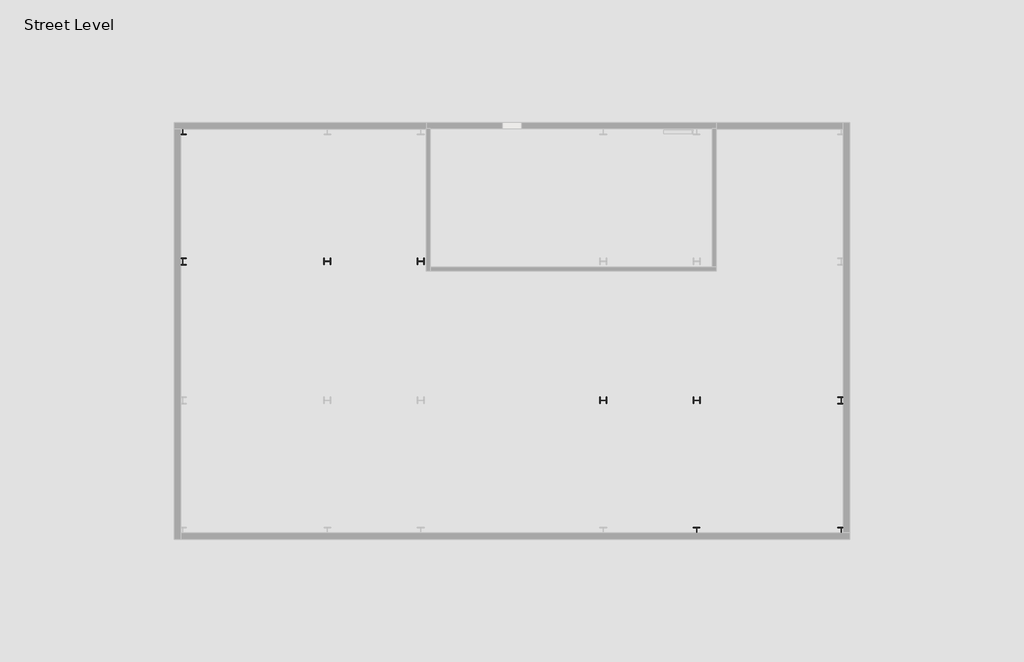
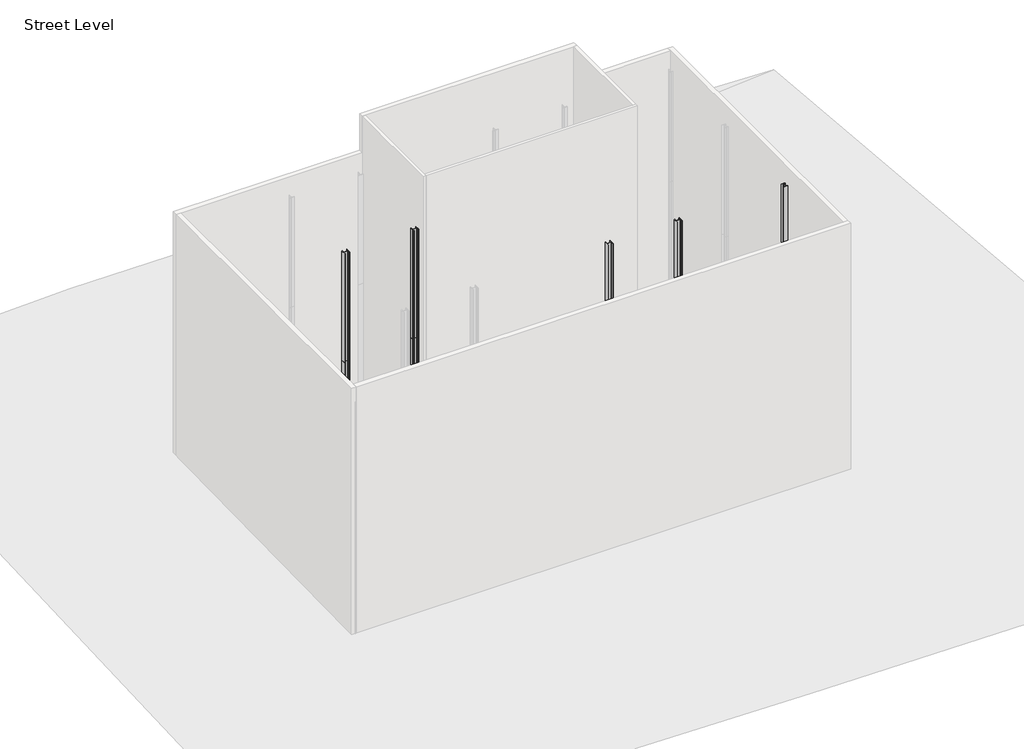
# One storey, part 2 of 3: 9 columns.
"""IFC4 building model written with IfcOpenShell, lengths in millimetres."""

from ifc_helpers import new_model, si_unit, point, frame, frame_2d, origin, place, context, project, spatial, polyline, circle_curve, trimmed, segment, composite_curve, outline, extrude, element, save

model = new_model("IFC4")

# Units and contexts
model_context = context("Model", 3, world=origin())
ifc_project = project(units=[si_unit("LENGTHUNIT", "METRE", prefix="MILLI")], contexts=[model_context])

# Site, building, storey
site = spatial("IfcSite", under=ifc_project)
building = spatial("IfcBuilding", under=site)
storey = spatial("IfcBuildingStorey", under=building, Name="Street Level", Elevation=-914.4)

# Columns
placement = place(None, origin())
element("IfcColumn", 1, ObjectType="W-Wide Flange-Column : W12X87", at=placement, inside=storey, context=model_context, shape_type="SweptSolid", body=[
    extrude(outline(composite_curve([segment(polyline([(3260.1377268, -3562.1684696), (3239.5637268, -3562.1684696), (3239.5637268, -3437.3274696)]), True, "CONTINUOUS"), segment(trimmed(circle_curve(frame_2d((3217.2752268, -3437.3274696)), 22.2885), [point((3239.5637268, -3437.3274696))], [point((3217.2752268, -3415.0389696))], True, "CARTESIAN"), True, "CONTINUOUS"), segment(polyline([(3217.2752268, -3415.0389696), (2985.5002268, -3415.0389696)]), True, "CONTINUOUS"), segment(trimmed(circle_curve(frame_2d((2985.5002268, -3437.3274696)), 22.2885), [point((2985.5002268, -3415.0389696))], [point((2963.2117268, -3437.3274696))], True, "CARTESIAN"), True, "CONTINUOUS"), segment(polyline([(2963.2117268, -3437.3274696), (2963.2117268, -3562.1684696), (2942.6377268, -3562.1684696), (2942.6377268, -3254.8284696), (2963.2117268, -3254.8284696), (2963.2117268, -3379.6694696)]), True, "CONTINUOUS"), segment(trimmed(circle_curve(frame_2d((2985.5002268, -3379.6694696)), 22.2885), [point((2963.2117268, -3379.6694696))], [point((2985.5002268, -3401.9579696))], True, "CARTESIAN"), True, "CONTINUOUS"), segment(polyline([(2985.5002268, -3401.9579696), (3217.2752268, -3401.9579696)]), True, "CONTINUOUS"), segment(trimmed(circle_curve(frame_2d((3217.2752268, -3379.6694696)), 22.2885), [point((3217.2752268, -3401.9579696))], [point((3239.5637268, -3379.6694696))], True, "CARTESIAN"), True, "CONTINUOUS"), segment(polyline([(3239.5637268, -3379.6694696), (3239.5637268, -3254.8284696), (3260.1377268, -3254.8284696), (3260.1377268, -3562.1684696)]), True, "CONTINUOUS")], self_intersect=False)), frame((0.0, 0.0, 7315.2), z_axis=(0.0, 0.0, 1.0), x_axis=(1.0, 0.0, 0.0)), (0.0, 0.0, 1.0), 7315.2),
    extrude(outline(composite_curve([segment(polyline([(3260.1377268, -3562.1684696), (3239.5637268, -3562.1684696), (3239.5637268, -3437.3274696)]), True, "CONTINUOUS"), segment(trimmed(circle_curve(frame_2d((3217.2752268, -3437.3274696)), 22.2885), [point((3239.5637268, -3437.3274696))], [point((3217.2752268, -3415.0389696))], True, "CARTESIAN"), True, "CONTINUOUS"), segment(polyline([(3217.2752268, -3415.0389696), (2985.5002268, -3415.0389696)]), True, "CONTINUOUS"), segment(trimmed(circle_curve(frame_2d((2985.5002268, -3437.3274696)), 22.2885), [point((2985.5002268, -3415.0389696))], [point((2963.2117268, -3437.3274696))], True, "CARTESIAN"), True, "CONTINUOUS"), segment(polyline([(2963.2117268, -3437.3274696), (2963.2117268, -3562.1684696), (2942.6377268, -3562.1684696), (2942.6377268, -3254.8284696), (2963.2117268, -3254.8284696), (2963.2117268, -3379.6694696)]), True, "CONTINUOUS"), segment(trimmed(circle_curve(frame_2d((2985.5002268, -3379.6694696)), 22.2885), [point((2963.2117268, -3379.6694696))], [point((2985.5002268, -3401.9579696))], True, "CARTESIAN"), True, "CONTINUOUS"), segment(polyline([(2985.5002268, -3401.9579696), (3217.2752268, -3401.9579696)]), True, "CONTINUOUS"), segment(trimmed(circle_curve(frame_2d((3217.2752268, -3379.6694696)), 22.2885), [point((3217.2752268, -3401.9579696))], [point((3239.5637268, -3379.6694696))], True, "CARTESIAN"), True, "CONTINUOUS"), segment(polyline([(3239.5637268, -3379.6694696), (3239.5637268, -3254.8284696), (3260.1377268, -3254.8284696), (3260.1377268, -3562.1684696)]), True, "CONTINUOUS")], self_intersect=False)), frame((0.0, 0.0, -914.4), z_axis=(0.0, 0.0, 1.0), x_axis=(1.0, 0.0, 0.0)), (0.0, 0.0, 1.0), 8229.6),
])
element("IfcColumn", 2, ObjectType="W-Wide Flange-Column : W12X87", at=placement, inside=storey, context=model_context, shape_type="SweptSolid", body=[
    extrude(outline(composite_curve([segment(polyline([(7628.9377268, -3562.1684696), (7608.3637268, -3562.1684696), (7608.3637268, -3437.3274696)]), True, "CONTINUOUS"), segment(trimmed(circle_curve(frame_2d((7586.0752268, -3437.3274696)), 22.2885), [point((7608.3637268, -3437.3274696))], [point((7586.0752268, -3415.0389696))], True, "CARTESIAN"), True, "CONTINUOUS"), segment(polyline([(7586.0752268, -3415.0389696), (7354.3002268, -3415.0389696)]), True, "CONTINUOUS"), segment(trimmed(circle_curve(frame_2d((7354.3002268, -3437.3274696)), 22.2885), [point((7354.3002268, -3415.0389696))], [point((7332.0117268, -3437.3274696))], True, "CARTESIAN"), True, "CONTINUOUS"), segment(polyline([(7332.0117268, -3437.3274696), (7332.0117268, -3562.1684696), (7311.4377268, -3562.1684696), (7311.4377268, -3254.8284696), (7332.0117268, -3254.8284696), (7332.0117268, -3379.6694696)]), True, "CONTINUOUS"), segment(trimmed(circle_curve(frame_2d((7354.3002268, -3379.6694696)), 22.2885), [point((7332.0117268, -3379.6694696))], [point((7354.3002268, -3401.9579696))], True, "CARTESIAN"), True, "CONTINUOUS"), segment(polyline([(7354.3002268, -3401.9579696), (7586.0752268, -3401.9579696)]), True, "CONTINUOUS"), segment(trimmed(circle_curve(frame_2d((7586.0752268, -3379.6694696)), 22.2885), [point((7586.0752268, -3401.9579696))], [point((7608.3637268, -3379.6694696))], True, "CARTESIAN"), True, "CONTINUOUS"), segment(polyline([(7608.3637268, -3379.6694696), (7608.3637268, -3254.8284696), (7628.9377268, -3254.8284696), (7628.9377268, -3562.1684696)]), True, "CONTINUOUS")], self_intersect=False)), frame((0.0, 0.0, 7315.2), z_axis=(0.0, 0.0, 1.0), x_axis=(1.0, 0.0, 0.0)), (0.0, 0.0, 1.0), 7315.2),
    extrude(outline(composite_curve([segment(polyline([(7628.9377268, -3562.1684696), (7608.3637268, -3562.1684696), (7608.3637268, -3437.3274696)]), True, "CONTINUOUS"), segment(trimmed(circle_curve(frame_2d((7586.0752268, -3437.3274696)), 22.2885), [point((7608.3637268, -3437.3274696))], [point((7586.0752268, -3415.0389696))], True, "CARTESIAN"), True, "CONTINUOUS"), segment(polyline([(7586.0752268, -3415.0389696), (7354.3002268, -3415.0389696)]), True, "CONTINUOUS"), segment(trimmed(circle_curve(frame_2d((7354.3002268, -3437.3274696)), 22.2885), [point((7354.3002268, -3415.0389696))], [point((7332.0117268, -3437.3274696))], True, "CARTESIAN"), True, "CONTINUOUS"), segment(polyline([(7332.0117268, -3437.3274696), (7332.0117268, -3562.1684696), (7311.4377268, -3562.1684696), (7311.4377268, -3254.8284696), (7332.0117268, -3254.8284696), (7332.0117268, -3379.6694696)]), True, "CONTINUOUS"), segment(trimmed(circle_curve(frame_2d((7354.3002268, -3379.6694696)), 22.2885), [point((7332.0117268, -3379.6694696))], [point((7354.3002268, -3401.9579696))], True, "CARTESIAN"), True, "CONTINUOUS"), segment(polyline([(7354.3002268, -3401.9579696), (7586.0752268, -3401.9579696)]), True, "CONTINUOUS"), segment(trimmed(circle_curve(frame_2d((7586.0752268, -3379.6694696)), 22.2885), [point((7586.0752268, -3401.9579696))], [point((7608.3637268, -3379.6694696))], True, "CARTESIAN"), True, "CONTINUOUS"), segment(polyline([(7608.3637268, -3379.6694696), (7608.3637268, -3254.8284696), (7628.9377268, -3254.8284696), (7628.9377268, -3562.1684696)]), True, "CONTINUOUS")], self_intersect=False)), frame((0.0, 0.0, -914.4), z_axis=(0.0, 0.0, 1.0), x_axis=(1.0, 0.0, 0.0)), (0.0, 0.0, 1.0), 8229.6),
])
element("IfcColumn", 3, ObjectType="W-Wide Flange-Column : W12X87", at=placement, inside=storey, context=model_context, shape_type="SweptSolid", body=[
    extrude(outline(composite_curve([segment(polyline([(-9643.0622732, 2940.2315304), (-9663.6362732, 2940.2315304), (-9663.6362732, 3065.0725304)]), True, "CONTINUOUS"), segment(trimmed(circle_curve(frame_2d((-9685.9247732, 3065.0725304)), 22.2885), [point((-9663.6362732, 3065.0725304))], [point((-9685.9247732, 3087.3610304))], True, "CARTESIAN"), True, "CONTINUOUS"), segment(polyline([(-9685.9247732, 3087.3610304), (-9917.6997732, 3087.3610304)]), True, "CONTINUOUS"), segment(trimmed(circle_curve(frame_2d((-9917.6997732, 3065.0725304)), 22.2885), [point((-9917.6997732, 3087.3610304))], [point((-9939.9882732, 3065.0725304))], True, "CARTESIAN"), True, "CONTINUOUS"), segment(polyline([(-9939.9882732, 3065.0725304), (-9939.9882732, 2940.2315304), (-9960.5622732, 2940.2315304), (-9960.5622732, 3247.5715304), (-9939.9882732, 3247.5715304), (-9939.9882732, 3122.7305304)]), True, "CONTINUOUS"), segment(trimmed(circle_curve(frame_2d((-9917.6997732, 3122.7305304)), 22.2885), [point((-9939.9882732, 3122.7305304))], [point((-9917.6997732, 3100.4420304))], True, "CARTESIAN"), True, "CONTINUOUS"), segment(polyline([(-9917.6997732, 3100.4420304), (-9685.9247732, 3100.4420304)]), True, "CONTINUOUS"), segment(trimmed(circle_curve(frame_2d((-9685.9247732, 3122.7305304)), 22.2885), [point((-9685.9247732, 3100.4420304))], [point((-9663.6362732, 3122.7305304))], True, "CARTESIAN"), True, "CONTINUOUS"), segment(polyline([(-9663.6362732, 3122.7305304), (-9663.6362732, 3247.5715304), (-9643.0622732, 3247.5715304), (-9643.0622732, 2940.2315304)]), True, "CONTINUOUS")], self_intersect=False)), frame((0.0, 0.0, 7315.2), z_axis=(0.0, 0.0, 1.0), x_axis=(1.0, 0.0, 0.0)), (0.0, 0.0, 1.0), 7315.2),
    extrude(outline(composite_curve([segment(polyline([(-9643.0622732, 2940.2315304), (-9663.6362732, 2940.2315304), (-9663.6362732, 3065.0725304)]), True, "CONTINUOUS"), segment(trimmed(circle_curve(frame_2d((-9685.9247732, 3065.0725304)), 22.2885), [point((-9663.6362732, 3065.0725304))], [point((-9685.9247732, 3087.3610304))], True, "CARTESIAN"), True, "CONTINUOUS"), segment(polyline([(-9685.9247732, 3087.3610304), (-9917.6997732, 3087.3610304)]), True, "CONTINUOUS"), segment(trimmed(circle_curve(frame_2d((-9917.6997732, 3065.0725304)), 22.2885), [point((-9917.6997732, 3087.3610304))], [point((-9939.9882732, 3065.0725304))], True, "CARTESIAN"), True, "CONTINUOUS"), segment(polyline([(-9939.9882732, 3065.0725304), (-9939.9882732, 2940.2315304), (-9960.5622732, 2940.2315304), (-9960.5622732, 3247.5715304), (-9939.9882732, 3247.5715304), (-9939.9882732, 3122.7305304)]), True, "CONTINUOUS"), segment(trimmed(circle_curve(frame_2d((-9917.6997732, 3122.7305304)), 22.2885), [point((-9939.9882732, 3122.7305304))], [point((-9917.6997732, 3100.4420304))], True, "CARTESIAN"), True, "CONTINUOUS"), segment(polyline([(-9917.6997732, 3100.4420304), (-9685.9247732, 3100.4420304)]), True, "CONTINUOUS"), segment(trimmed(circle_curve(frame_2d((-9685.9247732, 3122.7305304)), 22.2885), [point((-9685.9247732, 3100.4420304))], [point((-9663.6362732, 3122.7305304))], True, "CARTESIAN"), True, "CONTINUOUS"), segment(polyline([(-9663.6362732, 3122.7305304), (-9663.6362732, 3247.5715304), (-9643.0622732, 3247.5715304), (-9643.0622732, 2940.2315304)]), True, "CONTINUOUS")], self_intersect=False)), frame((0.0, 0.0, -914.4), z_axis=(0.0, 0.0, 1.0), x_axis=(1.0, 0.0, 0.0)), (0.0, 0.0, 1.0), 8229.6),
])
element("IfcColumn", 4, ObjectType="W-Wide Flange-Column : W12X87", at=placement, inside=storey, context=model_context, shape_type="SweptSolid", body=[
    extrude(outline(composite_curve([segment(polyline([(-5274.2622732, 2940.2315304), (-5294.8362732, 2940.2315304), (-5294.8362732, 3065.0725304)]), True, "CONTINUOUS"), segment(trimmed(circle_curve(frame_2d((-5317.1247732, 3065.0725304)), 22.2885), [point((-5294.8362732, 3065.0725304))], [point((-5317.1247732, 3087.3610304))], True, "CARTESIAN"), True, "CONTINUOUS"), segment(polyline([(-5317.1247732, 3087.3610304), (-5548.8997732, 3087.3610304)]), True, "CONTINUOUS"), segment(trimmed(circle_curve(frame_2d((-5548.8997732, 3065.0725304)), 22.2885), [point((-5548.8997732, 3087.3610304))], [point((-5571.1882732, 3065.0725304))], True, "CARTESIAN"), True, "CONTINUOUS"), segment(polyline([(-5571.1882732, 3065.0725304), (-5571.1882732, 2940.2315304), (-5591.7622732, 2940.2315304), (-5591.7622732, 3247.5715304), (-5571.1882732, 3247.5715304), (-5571.1882732, 3122.7305304)]), True, "CONTINUOUS"), segment(trimmed(circle_curve(frame_2d((-5548.8997732, 3122.7305304)), 22.2885), [point((-5571.1882732, 3122.7305304))], [point((-5548.8997732, 3100.4420304))], True, "CARTESIAN"), True, "CONTINUOUS"), segment(polyline([(-5548.8997732, 3100.4420304), (-5317.1247732, 3100.4420304)]), True, "CONTINUOUS"), segment(trimmed(circle_curve(frame_2d((-5317.1247732, 3122.7305304)), 22.2885), [point((-5317.1247732, 3100.4420304))], [point((-5294.8362732, 3122.7305304))], True, "CARTESIAN"), True, "CONTINUOUS"), segment(polyline([(-5294.8362732, 3122.7305304), (-5294.8362732, 3247.5715304), (-5274.2622732, 3247.5715304), (-5274.2622732, 2940.2315304)]), True, "CONTINUOUS")], self_intersect=False)), frame((0.0, 0.0, 7315.2), z_axis=(0.0, 0.0, 1.0), x_axis=(1.0, 0.0, 0.0)), (0.0, 0.0, 1.0), 7315.2),
    extrude(outline(composite_curve([segment(polyline([(-5274.2622732, 2940.2315304), (-5294.8362732, 2940.2315304), (-5294.8362732, 3065.0725304)]), True, "CONTINUOUS"), segment(trimmed(circle_curve(frame_2d((-5317.1247732, 3065.0725304)), 22.2885), [point((-5294.8362732, 3065.0725304))], [point((-5317.1247732, 3087.3610304))], True, "CARTESIAN"), True, "CONTINUOUS"), segment(polyline([(-5317.1247732, 3087.3610304), (-5548.8997732, 3087.3610304)]), True, "CONTINUOUS"), segment(trimmed(circle_curve(frame_2d((-5548.8997732, 3065.0725304)), 22.2885), [point((-5548.8997732, 3087.3610304))], [point((-5571.1882732, 3065.0725304))], True, "CARTESIAN"), True, "CONTINUOUS"), segment(polyline([(-5571.1882732, 3065.0725304), (-5571.1882732, 2940.2315304), (-5591.7622732, 2940.2315304), (-5591.7622732, 3247.5715304), (-5571.1882732, 3247.5715304), (-5571.1882732, 3122.7305304)]), True, "CONTINUOUS"), segment(trimmed(circle_curve(frame_2d((-5548.8997732, 3122.7305304)), 22.2885), [point((-5571.1882732, 3122.7305304))], [point((-5548.8997732, 3100.4420304))], True, "CARTESIAN"), True, "CONTINUOUS"), segment(polyline([(-5548.8997732, 3100.4420304), (-5317.1247732, 3100.4420304)]), True, "CONTINUOUS"), segment(trimmed(circle_curve(frame_2d((-5317.1247732, 3122.7305304)), 22.2885), [point((-5317.1247732, 3100.4420304))], [point((-5294.8362732, 3122.7305304))], True, "CARTESIAN"), True, "CONTINUOUS"), segment(polyline([(-5294.8362732, 3122.7305304), (-5294.8362732, 3247.5715304), (-5274.2622732, 3247.5715304), (-5274.2622732, 2940.2315304)]), True, "CONTINUOUS")], self_intersect=False)), frame((0.0, 0.0, -914.4), z_axis=(0.0, 0.0, 1.0), x_axis=(1.0, 0.0, 0.0)), (0.0, 0.0, 1.0), 8229.6),
])
element("IfcColumn", 5, ObjectType="W-Wide Flange-Column : W12X87", at=placement, inside=storey, context=model_context, shape_type="SweptSolid", body=[
    extrude(outline(composite_curve([segment(polyline([(-16404.5422732, 9348.6515304), (-16404.5422732, 9328.0775304), (-16529.3832732, 9328.0775304)]), True, "CONTINUOUS"), segment(trimmed(circle_curve(frame_2d((-16529.3832732, 9305.7890304)), 22.2885), [point((-16529.3832732, 9328.0775304))], [point((-16551.6717732, 9305.7890304))], True, "CARTESIAN"), True, "CONTINUOUS"), segment(polyline([(-16551.6717732, 9305.7890304), (-16551.6717732, 9074.0140304)]), True, "CONTINUOUS"), segment(trimmed(circle_curve(frame_2d((-16529.3832732, 9074.0140304)), 22.2885), [point((-16551.6717732, 9074.0140304))], [point((-16529.3832732, 9051.7255304))], True, "CARTESIAN"), True, "CONTINUOUS"), segment(polyline([(-16529.3832732, 9051.7255304), (-16404.5422732, 9051.7255304), (-16404.5422732, 9031.1515304), (-16711.8822732, 9031.1515304), (-16711.8822732, 9051.7255304), (-16587.0412732, 9051.7255304)]), True, "CONTINUOUS"), segment(trimmed(circle_curve(frame_2d((-16587.0412732, 9074.0140304)), 22.2885), [point((-16587.0412732, 9051.7255304))], [point((-16564.7527732, 9074.0140304))], True, "CARTESIAN"), True, "CONTINUOUS"), segment(polyline([(-16564.7527732, 9074.0140304), (-16564.7527732, 9305.7890304)]), True, "CONTINUOUS"), segment(trimmed(circle_curve(frame_2d((-16587.0412732, 9305.7890304)), 22.2885), [point((-16564.7527732, 9305.7890304))], [point((-16587.0412732, 9328.0775304))], True, "CARTESIAN"), True, "CONTINUOUS"), segment(polyline([(-16587.0412732, 9328.0775304), (-16711.8822732, 9328.0775304), (-16711.8822732, 9348.6515304), (-16404.5422732, 9348.6515304)]), True, "CONTINUOUS")], self_intersect=False)), frame((0.0, 0.0, 7315.2), z_axis=(0.0, 0.0, 1.0), x_axis=(1.0, 0.0, 0.0)), (0.0, 0.0, 1.0), 7315.2),
    extrude(outline(composite_curve([segment(polyline([(-16404.5422732, 9348.6515304), (-16404.5422732, 9328.0775304), (-16529.3832732, 9328.0775304)]), True, "CONTINUOUS"), segment(trimmed(circle_curve(frame_2d((-16529.3832732, 9305.7890304)), 22.2885), [point((-16529.3832732, 9328.0775304))], [point((-16551.6717732, 9305.7890304))], True, "CARTESIAN"), True, "CONTINUOUS"), segment(polyline([(-16551.6717732, 9305.7890304), (-16551.6717732, 9074.0140304)]), True, "CONTINUOUS"), segment(trimmed(circle_curve(frame_2d((-16529.3832732, 9074.0140304)), 22.2885), [point((-16551.6717732, 9074.0140304))], [point((-16529.3832732, 9051.7255304))], True, "CARTESIAN"), True, "CONTINUOUS"), segment(polyline([(-16529.3832732, 9051.7255304), (-16404.5422732, 9051.7255304), (-16404.5422732, 9031.1515304), (-16711.8822732, 9031.1515304), (-16711.8822732, 9051.7255304), (-16587.0412732, 9051.7255304)]), True, "CONTINUOUS"), segment(trimmed(circle_curve(frame_2d((-16587.0412732, 9074.0140304)), 22.2885), [point((-16587.0412732, 9051.7255304))], [point((-16564.7527732, 9074.0140304))], True, "CARTESIAN"), True, "CONTINUOUS"), segment(polyline([(-16564.7527732, 9074.0140304), (-16564.7527732, 9305.7890304)]), True, "CONTINUOUS"), segment(trimmed(circle_curve(frame_2d((-16587.0412732, 9305.7890304)), 22.2885), [point((-16564.7527732, 9305.7890304))], [point((-16587.0412732, 9328.0775304))], True, "CARTESIAN"), True, "CONTINUOUS"), segment(polyline([(-16587.0412732, 9328.0775304), (-16711.8822732, 9328.0775304), (-16711.8822732, 9348.6515304), (-16404.5422732, 9348.6515304)]), True, "CONTINUOUS")], self_intersect=False)), frame((0.0, 0.0, -914.4), z_axis=(0.0, 0.0, 1.0), x_axis=(1.0, 0.0, 0.0)), (0.0, 0.0, 1.0), 8229.6),
])
element("IfcColumn", 6, ObjectType="W-Wide Flange-Column : W12X87", at=placement, inside=storey, context=model_context, shape_type="SweptSolid", body=[
    extrude(outline(composite_curve([segment(polyline([(-16404.5422732, 3252.6515304), (-16404.5422732, 3232.0775304), (-16529.3832732, 3232.0775304)]), True, "CONTINUOUS"), segment(trimmed(circle_curve(frame_2d((-16529.3832732, 3209.7890304)), 22.2885), [point((-16529.3832732, 3232.0775304))], [point((-16551.6717732, 3209.7890304))], True, "CARTESIAN"), True, "CONTINUOUS"), segment(polyline([(-16551.6717732, 3209.7890304), (-16551.6717732, 2978.0140304)]), True, "CONTINUOUS"), segment(trimmed(circle_curve(frame_2d((-16529.3832732, 2978.0140304)), 22.2885), [point((-16551.6717732, 2978.0140304))], [point((-16529.3832732, 2955.7255304))], True, "CARTESIAN"), True, "CONTINUOUS"), segment(polyline([(-16529.3832732, 2955.7255304), (-16404.5422732, 2955.7255304), (-16404.5422732, 2935.1515304), (-16711.8822732, 2935.1515304), (-16711.8822732, 2955.7255304), (-16587.0412732, 2955.7255304)]), True, "CONTINUOUS"), segment(trimmed(circle_curve(frame_2d((-16587.0412732, 2978.0140304)), 22.2885), [point((-16587.0412732, 2955.7255304))], [point((-16564.7527732, 2978.0140304))], True, "CARTESIAN"), True, "CONTINUOUS"), segment(polyline([(-16564.7527732, 2978.0140304), (-16564.7527732, 3209.7890304)]), True, "CONTINUOUS"), segment(trimmed(circle_curve(frame_2d((-16587.0412732, 3209.7890304)), 22.2885), [point((-16564.7527732, 3209.7890304))], [point((-16587.0412732, 3232.0775304))], True, "CARTESIAN"), True, "CONTINUOUS"), segment(polyline([(-16587.0412732, 3232.0775304), (-16711.8822732, 3232.0775304), (-16711.8822732, 3252.6515304), (-16404.5422732, 3252.6515304)]), True, "CONTINUOUS")], self_intersect=False)), frame((0.0, 0.0, 7315.2), z_axis=(0.0, 0.0, 1.0), x_axis=(1.0, 0.0, 0.0)), (0.0, 0.0, 1.0), 7315.2),
    extrude(outline(composite_curve([segment(polyline([(-16404.5422732, 3252.6515304), (-16404.5422732, 3232.0775304), (-16529.3832732, 3232.0775304)]), True, "CONTINUOUS"), segment(trimmed(circle_curve(frame_2d((-16529.3832732, 3209.7890304)), 22.2885), [point((-16529.3832732, 3232.0775304))], [point((-16551.6717732, 3209.7890304))], True, "CARTESIAN"), True, "CONTINUOUS"), segment(polyline([(-16551.6717732, 3209.7890304), (-16551.6717732, 2978.0140304)]), True, "CONTINUOUS"), segment(trimmed(circle_curve(frame_2d((-16529.3832732, 2978.0140304)), 22.2885), [point((-16551.6717732, 2978.0140304))], [point((-16529.3832732, 2955.7255304))], True, "CARTESIAN"), True, "CONTINUOUS"), segment(polyline([(-16529.3832732, 2955.7255304), (-16404.5422732, 2955.7255304), (-16404.5422732, 2935.1515304), (-16711.8822732, 2935.1515304), (-16711.8822732, 2955.7255304), (-16587.0412732, 2955.7255304)]), True, "CONTINUOUS"), segment(trimmed(circle_curve(frame_2d((-16587.0412732, 2978.0140304)), 22.2885), [point((-16587.0412732, 2955.7255304))], [point((-16564.7527732, 2978.0140304))], True, "CARTESIAN"), True, "CONTINUOUS"), segment(polyline([(-16564.7527732, 2978.0140304), (-16564.7527732, 3209.7890304)]), True, "CONTINUOUS"), segment(trimmed(circle_curve(frame_2d((-16587.0412732, 3209.7890304)), 22.2885), [point((-16564.7527732, 3209.7890304))], [point((-16587.0412732, 3232.0775304))], True, "CARTESIAN"), True, "CONTINUOUS"), segment(polyline([(-16587.0412732, 3232.0775304), (-16711.8822732, 3232.0775304), (-16711.8822732, 3252.6515304), (-16404.5422732, 3252.6515304)]), True, "CONTINUOUS")], self_intersect=False)), frame((0.0, 0.0, -914.4), z_axis=(0.0, 0.0, 1.0), x_axis=(1.0, 0.0, 0.0)), (0.0, 0.0, 1.0), 8229.6),
])
element("IfcColumn", 7, ObjectType="W-Wide Flange-Column : W12X87", at=placement, inside=storey, context=model_context, shape_type="SweptSolid", body=[
    extrude(outline(composite_curve([segment(polyline([(14380.2577268, -3249.7484696), (14380.2577268, -3270.3224696), (14255.4167268, -3270.3224696)]), True, "CONTINUOUS"), segment(trimmed(circle_curve(frame_2d((14255.4167268, -3292.6109696)), 22.2885), [point((14255.4167268, -3270.3224696))], [point((14233.1282268, -3292.6109696))], True, "CARTESIAN"), True, "CONTINUOUS"), segment(polyline([(14233.1282268, -3292.6109696), (14233.1282268, -3524.3859696)]), True, "CONTINUOUS"), segment(trimmed(circle_curve(frame_2d((14255.4167268, -3524.3859696)), 22.2885), [point((14233.1282268, -3524.3859696))], [point((14255.4167268, -3546.6744696))], True, "CARTESIAN"), True, "CONTINUOUS"), segment(polyline([(14255.4167268, -3546.6744696), (14380.2577268, -3546.6744696), (14380.2577268, -3567.2484696), (14072.9177268, -3567.2484696), (14072.9177268, -3546.6744696), (14197.7587268, -3546.6744696)]), True, "CONTINUOUS"), segment(trimmed(circle_curve(frame_2d((14197.7587268, -3524.3859696)), 22.2885), [point((14197.7587268, -3546.6744696))], [point((14220.0472268, -3524.3859696))], True, "CARTESIAN"), True, "CONTINUOUS"), segment(polyline([(14220.0472268, -3524.3859696), (14220.0472268, -3292.6109696)]), True, "CONTINUOUS"), segment(trimmed(circle_curve(frame_2d((14197.7587268, -3292.6109696)), 22.2885), [point((14220.0472268, -3292.6109696))], [point((14197.7587268, -3270.3224696))], True, "CARTESIAN"), True, "CONTINUOUS"), segment(polyline([(14197.7587268, -3270.3224696), (14072.9177268, -3270.3224696), (14072.9177268, -3249.7484696), (14380.2577268, -3249.7484696)]), True, "CONTINUOUS")], self_intersect=False)), frame((0.0, 0.0, 7315.2), z_axis=(0.0, 0.0, 1.0), x_axis=(1.0, 0.0, 0.0)), (0.0, 0.0, 1.0), 7315.2),
    extrude(outline(composite_curve([segment(polyline([(14380.2577268, -3249.7484696), (14380.2577268, -3270.3224696), (14255.4167268, -3270.3224696)]), True, "CONTINUOUS"), segment(trimmed(circle_curve(frame_2d((14255.4167268, -3292.6109696)), 22.2885), [point((14255.4167268, -3270.3224696))], [point((14233.1282268, -3292.6109696))], True, "CARTESIAN"), True, "CONTINUOUS"), segment(polyline([(14233.1282268, -3292.6109696), (14233.1282268, -3524.3859696)]), True, "CONTINUOUS"), segment(trimmed(circle_curve(frame_2d((14255.4167268, -3524.3859696)), 22.2885), [point((14233.1282268, -3524.3859696))], [point((14255.4167268, -3546.6744696))], True, "CARTESIAN"), True, "CONTINUOUS"), segment(polyline([(14255.4167268, -3546.6744696), (14380.2577268, -3546.6744696), (14380.2577268, -3567.2484696), (14072.9177268, -3567.2484696), (14072.9177268, -3546.6744696), (14197.7587268, -3546.6744696)]), True, "CONTINUOUS"), segment(trimmed(circle_curve(frame_2d((14197.7587268, -3524.3859696)), 22.2885), [point((14197.7587268, -3546.6744696))], [point((14220.0472268, -3524.3859696))], True, "CARTESIAN"), True, "CONTINUOUS"), segment(polyline([(14220.0472268, -3524.3859696), (14220.0472268, -3292.6109696)]), True, "CONTINUOUS"), segment(trimmed(circle_curve(frame_2d((14197.7587268, -3292.6109696)), 22.2885), [point((14220.0472268, -3292.6109696))], [point((14197.7587268, -3270.3224696))], True, "CARTESIAN"), True, "CONTINUOUS"), segment(polyline([(14197.7587268, -3270.3224696), (14072.9177268, -3270.3224696), (14072.9177268, -3249.7484696), (14380.2577268, -3249.7484696)]), True, "CONTINUOUS")], self_intersect=False)), frame((0.0, 0.0, -914.4), z_axis=(0.0, 0.0, 1.0), x_axis=(1.0, 0.0, 0.0)), (0.0, 0.0, 1.0), 8229.6),
])
element("IfcColumn", 8, ObjectType="W-Wide Flange-Column : W12X87", at=placement, inside=storey, context=model_context, shape_type="SweptSolid", body=[
    extrude(outline(composite_curve([segment(polyline([(14380.2577268, -9345.7484696), (14380.2577268, -9366.3224696), (14255.4167268, -9366.3224696)]), True, "CONTINUOUS"), segment(trimmed(circle_curve(frame_2d((14255.4167268, -9388.6109696)), 22.2885), [point((14255.4167268, -9366.3224696))], [point((14233.1282268, -9388.6109696))], True, "CARTESIAN"), True, "CONTINUOUS"), segment(polyline([(14233.1282268, -9388.6109696), (14233.1282268, -9620.3859696)]), True, "CONTINUOUS"), segment(trimmed(circle_curve(frame_2d((14255.4167268, -9620.3859696)), 22.2885), [point((14233.1282268, -9620.3859696))], [point((14255.4167268, -9642.6744696))], True, "CARTESIAN"), True, "CONTINUOUS"), segment(polyline([(14255.4167268, -9642.6744696), (14380.2577268, -9642.6744696), (14380.2577268, -9663.2484696), (14072.9177268, -9663.2484696), (14072.9177268, -9642.6744696), (14197.7587268, -9642.6744696)]), True, "CONTINUOUS"), segment(trimmed(circle_curve(frame_2d((14197.7587268, -9620.3859696)), 22.2885), [point((14197.7587268, -9642.6744696))], [point((14220.0472268, -9620.3859696))], True, "CARTESIAN"), True, "CONTINUOUS"), segment(polyline([(14220.0472268, -9620.3859696), (14220.0472268, -9388.6109696)]), True, "CONTINUOUS"), segment(trimmed(circle_curve(frame_2d((14197.7587268, -9388.6109696)), 22.2885), [point((14220.0472268, -9388.6109696))], [point((14197.7587268, -9366.3224696))], True, "CARTESIAN"), True, "CONTINUOUS"), segment(polyline([(14197.7587268, -9366.3224696), (14072.9177268, -9366.3224696), (14072.9177268, -9345.7484696), (14380.2577268, -9345.7484696)]), True, "CONTINUOUS")], self_intersect=False)), frame((0.0, 0.0, 7315.2), z_axis=(0.0, 0.0, 1.0), x_axis=(1.0, 0.0, 0.0)), (0.0, 0.0, 1.0), 7315.2),
    extrude(outline(composite_curve([segment(polyline([(14380.2577268, -9345.7484696), (14380.2577268, -9366.3224696), (14255.4167268, -9366.3224696)]), True, "CONTINUOUS"), segment(trimmed(circle_curve(frame_2d((14255.4167268, -9388.6109696)), 22.2885), [point((14255.4167268, -9366.3224696))], [point((14233.1282268, -9388.6109696))], True, "CARTESIAN"), True, "CONTINUOUS"), segment(polyline([(14233.1282268, -9388.6109696), (14233.1282268, -9620.3859696)]), True, "CONTINUOUS"), segment(trimmed(circle_curve(frame_2d((14255.4167268, -9620.3859696)), 22.2885), [point((14233.1282268, -9620.3859696))], [point((14255.4167268, -9642.6744696))], True, "CARTESIAN"), True, "CONTINUOUS"), segment(polyline([(14255.4167268, -9642.6744696), (14380.2577268, -9642.6744696), (14380.2577268, -9663.2484696), (14072.9177268, -9663.2484696), (14072.9177268, -9642.6744696), (14197.7587268, -9642.6744696)]), True, "CONTINUOUS"), segment(trimmed(circle_curve(frame_2d((14197.7587268, -9620.3859696)), 22.2885), [point((14197.7587268, -9642.6744696))], [point((14220.0472268, -9620.3859696))], True, "CARTESIAN"), True, "CONTINUOUS"), segment(polyline([(14220.0472268, -9620.3859696), (14220.0472268, -9388.6109696)]), True, "CONTINUOUS"), segment(trimmed(circle_curve(frame_2d((14197.7587268, -9388.6109696)), 22.2885), [point((14220.0472268, -9388.6109696))], [point((14197.7587268, -9366.3224696))], True, "CARTESIAN"), True, "CONTINUOUS"), segment(polyline([(14197.7587268, -9366.3224696), (14072.9177268, -9366.3224696), (14072.9177268, -9345.7484696), (14380.2577268, -9345.7484696)]), True, "CONTINUOUS")], self_intersect=False)), frame((0.0, 0.0, -914.4), z_axis=(0.0, 0.0, 1.0), x_axis=(1.0, 0.0, 0.0)), (0.0, 0.0, 1.0), 8229.6),
])
element("IfcColumn", 9, ObjectType="W-Wide Flange-Column : W12X87", at=placement, inside=storey, context=model_context, shape_type="SweptSolid", body=[
    extrude(outline(composite_curve([segment(polyline([(7623.8577268, -9345.7484696), (7623.8577268, -9366.3224696), (7499.0167268, -9366.3224696)]), True, "CONTINUOUS"), segment(trimmed(circle_curve(frame_2d((7499.0167268, -9388.6109696)), 22.2885), [point((7499.0167268, -9366.3224696))], [point((7476.7282268, -9388.6109696))], True, "CARTESIAN"), True, "CONTINUOUS"), segment(polyline([(7476.7282268, -9388.6109696), (7476.7282268, -9620.3859696)]), True, "CONTINUOUS"), segment(trimmed(circle_curve(frame_2d((7499.0167268, -9620.3859696)), 22.2885), [point((7476.7282268, -9620.3859696))], [point((7499.0167268, -9642.6744696))], True, "CARTESIAN"), True, "CONTINUOUS"), segment(polyline([(7499.0167268, -9642.6744696), (7623.8577268, -9642.6744696), (7623.8577268, -9663.2484696), (7316.5177268, -9663.2484696), (7316.5177268, -9642.6744696), (7441.3587268, -9642.6744696)]), True, "CONTINUOUS"), segment(trimmed(circle_curve(frame_2d((7441.3587268, -9620.3859696)), 22.2885), [point((7441.3587268, -9642.6744696))], [point((7463.6472268, -9620.3859696))], True, "CARTESIAN"), True, "CONTINUOUS"), segment(polyline([(7463.6472268, -9620.3859696), (7463.6472268, -9388.6109696)]), True, "CONTINUOUS"), segment(trimmed(circle_curve(frame_2d((7441.3587268, -9388.6109696)), 22.2885), [point((7463.6472268, -9388.6109696))], [point((7441.3587268, -9366.3224696))], True, "CARTESIAN"), True, "CONTINUOUS"), segment(polyline([(7441.3587268, -9366.3224696), (7316.5177268, -9366.3224696), (7316.5177268, -9345.7484696), (7623.8577268, -9345.7484696)]), True, "CONTINUOUS")], self_intersect=False)), frame((0.0, 0.0, 7315.2), z_axis=(0.0, 0.0, 1.0), x_axis=(1.0, 0.0, 0.0)), (0.0, 0.0, 1.0), 7315.2),
    extrude(outline(composite_curve([segment(polyline([(7623.8577268, -9345.7484696), (7623.8577268, -9366.3224696), (7499.0167268, -9366.3224696)]), True, "CONTINUOUS"), segment(trimmed(circle_curve(frame_2d((7499.0167268, -9388.6109696)), 22.2885), [point((7499.0167268, -9366.3224696))], [point((7476.7282268, -9388.6109696))], True, "CARTESIAN"), True, "CONTINUOUS"), segment(polyline([(7476.7282268, -9388.6109696), (7476.7282268, -9620.3859696)]), True, "CONTINUOUS"), segment(trimmed(circle_curve(frame_2d((7499.0167268, -9620.3859696)), 22.2885), [point((7476.7282268, -9620.3859696))], [point((7499.0167268, -9642.6744696))], True, "CARTESIAN"), True, "CONTINUOUS"), segment(polyline([(7499.0167268, -9642.6744696), (7623.8577268, -9642.6744696), (7623.8577268, -9663.2484696), (7316.5177268, -9663.2484696), (7316.5177268, -9642.6744696), (7441.3587268, -9642.6744696)]), True, "CONTINUOUS"), segment(trimmed(circle_curve(frame_2d((7441.3587268, -9620.3859696)), 22.2885), [point((7441.3587268, -9642.6744696))], [point((7463.6472268, -9620.3859696))], True, "CARTESIAN"), True, "CONTINUOUS"), segment(polyline([(7463.6472268, -9620.3859696), (7463.6472268, -9388.6109696)]), True, "CONTINUOUS"), segment(trimmed(circle_curve(frame_2d((7441.3587268, -9388.6109696)), 22.2885), [point((7463.6472268, -9388.6109696))], [point((7441.3587268, -9366.3224696))], True, "CARTESIAN"), True, "CONTINUOUS"), segment(polyline([(7441.3587268, -9366.3224696), (7316.5177268, -9366.3224696), (7316.5177268, -9345.7484696), (7623.8577268, -9345.7484696)]), True, "CONTINUOUS")], self_intersect=False)), frame((0.0, 0.0, -914.4), z_axis=(0.0, 0.0, 1.0), x_axis=(1.0, 0.0, 0.0)), (0.0, 0.0, 1.0), 8229.6),
])

save(model, "model.ifc")

# Revit data of these elements
# Type "W-Wide Flange-Column : W12X87"
#   Assembly Code = "B10"
#   W = 87
#   bf = 1' - 0.1"
#   d = 1' - 0 1/2"
#   k = 0' - 1 11/16"
#   kr = 0' - 0.8775"
#   tf = 0' - 0.81"
#   tw = 0' - 0.515"
#   A = 0.177778 SF
#   Structural Material [instance default] = Steel ASTM A992
# Elements 1, 2, 3, 4, 5, 6, 7, 8, 9 (IfcColumn, "W-Wide Flange-Column : W12X87")
#   Structural Material = Steel ASTM A992
#   Phase Created = New Construction
#   Materials on its faces: "Steel ASTM A992"
# Materials
#   "Steel ASTM A992": class "Metal", colour RGB 199 199 199, transparency 0, Description = "Structural steel 50ksi", Cost = 0
